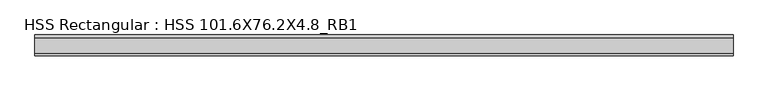
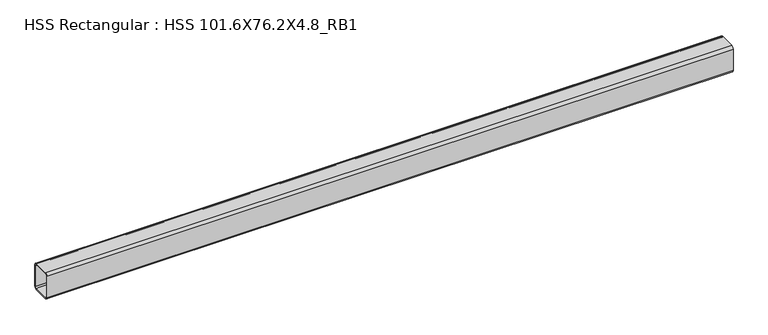
"""IFC4 building model written with IfcOpenShell, lengths in millimetres: beam geometry, HSS Rectangular : HSS 101.6X76.2X4.8_RB1."""

import ifcopenshell
import ifcopenshell.guid

model = None  # the IFC model being written
_history = None  # IfcOwnerHistory: only IFC2X3 demands one
_inside = {}  # id of a spatial element -> (the spatial element, [elements in it])
_under = {}  # id of a project, library or spatial element -> (it, [spatial elements below it])
_declared = {}  # id of a project -> (the project, [libraries it declares])
_typed = {}  # id of a type object -> (the type object, [elements of that type])
_made_of = {}  # id of a material, layer set ... -> (it, [elements and type objects made of it])


def new_model(schema):
    """Start an empty IFC model of exactly this schema.

    Asked for "IFC4X3", IfcOpenShell would pick the latest addendum, in which some entities
    have other attributes; the version numbers below select the first issue.
    IFC2X3 requires an IfcOwnerHistory on every rooted entity: one is made here for all.
    """
    global model, _history
    if schema == "IFC4X3":
        model = ifcopenshell.file(schema_version=(4, 3, 0, 0))
    else:
        model = ifcopenshell.file(schema=schema)
    _inside.clear()
    _under.clear()
    _declared.clear()
    _typed.clear()
    _made_of.clear()
    _history = None
    if model.schema == "IFC2X3":
        org = make("IfcOrganization", Name="unknown")
        user = make(
            "IfcPersonAndOrganization",
            ThePerson=make("IfcPerson", FamilyName="unknown"),
            TheOrganization=org,
        )
        app = make(
            "IfcApplication",
            ApplicationDeveloper=org,
            Version="unknown",
            ApplicationFullName="unknown",
            ApplicationIdentifier="unknown",
        )
        _history = make(
            "IfcOwnerHistory",
            OwningUser=user,
            OwningApplication=app,
            ChangeAction="ADDED",
            CreationDate=0,
        )
    return model


def make(cls, **values):
    """One entity of the class cls with the attributes given. An attribute that is None is left unset."""
    return model.create_entity(
        cls, **{name: value for name, value in values.items() if value is not None}
    )


def rooted(cls, **values):
    """An entity with a GlobalId (a new one), such as an element, a storey or a relation."""
    return make(cls, GlobalId=ifcopenshell.guid.new(), OwnerHistory=_history, **values)


def si_unit(unit_type, name, prefix=None):
    """IfcSIUnit, for example si_unit("LENGTHUNIT", "METRE", prefix="MILLI")."""
    return make("IfcSIUnit", UnitType=unit_type, Prefix=prefix, Name=name)


def assignment(units):
    """IfcUnitAssignment: the units of a project."""
    return None if units is None else make("IfcUnitAssignment", Units=units)


def point(xyz):
    """IfcCartesianPoint."""
    return None if xyz is None else make("IfcCartesianPoint", Coordinates=xyz)


def direction(xyz):
    """IfcDirection."""
    return None if xyz is None else make("IfcDirection", DirectionRatios=xyz)


def frame(location, z_axis=None, x_axis=None):
    """IfcAxis2Placement3D, a coordinate frame: its origin and axes. An axis left out is left unset."""
    return make(
        "IfcAxis2Placement3D",
        Location=point(location),
        Axis=direction(z_axis),
        RefDirection=direction(x_axis),
    )


def frame_2d(location, x_axis=None):
    """IfcAxis2Placement2D, a coordinate frame in the plane: its origin and x axis."""
    return make(
        "IfcAxis2Placement2D", Location=point(location), RefDirection=direction(x_axis)
    )


def origin():
    """The frame at (0, 0, 0) with its axes left unset."""
    return frame((0.0, 0.0, 0.0))


def place(relative_to, where):
    """IfcLocalPlacement: puts the frame where relative to a parent placement (None: the world)."""
    return make(
        "IfcLocalPlacement", PlacementRelTo=relative_to, RelativePlacement=where
    )


def context(
    kind, dimensions, precision=None, world=None, true_north=None, identifier=None
):
    """IfcGeometricRepresentationContext, for example the 3D "Model" context."""
    return make(
        "IfcGeometricRepresentationContext",
        ContextIdentifier=identifier,
        ContextType=kind,
        CoordinateSpaceDimension=dimensions,
        Precision=precision,
        WorldCoordinateSystem=world,
        TrueNorth=true_north,
    )


def project(units=None, contexts=None):
    """IfcProject with its units and contexts."""
    return rooted(
        "IfcProject",
        Name="project",
        RepresentationContexts=contexts,
        UnitsInContext=assignment(units),
    )


def spatial(cls, under=None, at=None, **own):
    """A site, building, storey or space (cls), placed at a placement, below another one or the project."""
    s = rooted(cls, ObjectPlacement=at, **own)
    if under is not None:
        _under.setdefault(under.id(), (under, []))[1].append(s)
    return s


def polyline(points):
    """IfcPolyline through the points."""
    return make("IfcPolyline", Points=[point(p) for p in points])


def circle_curve(where, radius):
    """IfcCircle in the frame where."""
    return make("IfcCircle", Position=where, Radius=radius)


def trimmed(basis, trim1, trim2, sense, master):
    """IfcTrimmedCurve: the piece of a basis curve between two trims."""
    return make(
        "IfcTrimmedCurve",
        BasisCurve=basis,
        Trim1=trim1,
        Trim2=trim2,
        SenseAgreement=sense,
        MasterRepresentation=master,
    )


def segment(curve, same_sense, transition):
    """IfcCompositeCurveSegment."""
    return make(
        "IfcCompositeCurveSegment",
        Transition=transition,
        SameSense=same_sense,
        ParentCurve=curve,
    )


def composite_curve(segments, self_intersect=None):
    """IfcCompositeCurve: segments joined end to end."""
    return make("IfcCompositeCurve", Segments=segments, SelfIntersect=self_intersect)


def outline(outer, holes=None, kind="AREA"):
    """IfcArbitraryClosedProfileDef: a profile drawn as a closed curve; with holes, ...WithVoids."""
    if holes is None:
        return make("IfcArbitraryClosedProfileDef", ProfileType=kind, OuterCurve=outer)
    return make(
        "IfcArbitraryProfileDefWithVoids",
        ProfileType=kind,
        OuterCurve=outer,
        InnerCurves=holes,
    )


def extrude(swept, where, along, depth):
    """IfcExtrudedAreaSolid: the profile swept, set in the frame where, extruded along a direction by depth."""
    return make(
        "IfcExtrudedAreaSolid",
        SweptArea=swept,
        Position=where,
        ExtrudedDirection=direction(along),
        Depth=depth,
    )


def shape(context_of_items, identifier, shape_type, items):
    """IfcShapeRepresentation: the items that make up one representation, for example the "Body"."""
    return make(
        "IfcShapeRepresentation",
        ContextOfItems=context_of_items,
        RepresentationIdentifier=identifier,
        RepresentationType=shape_type,
        Items=items,
    )


def source(mapping_origin, context_of_items, identifier, shape_type, items):
    """IfcRepresentationMap: a shape defined once, which mapped items show again and again."""
    return make(
        "IfcRepresentationMap",
        MappingOrigin=mapping_origin,
        MappedRepresentation=shape(context_of_items, identifier, shape_type, items),
    )


def transform(
    local_origin,
    x_axis=None,
    y_axis=None,
    z_axis=None,
    scale=None,
    scale2=None,
    scale3=None,
    uniform=True,
):
    """IfcCartesianTransformationOperator3D, or its non-uniform kind. x_axis, y_axis, z_axis: its Axis1, 2, 3."""
    if uniform:
        return make(
            "IfcCartesianTransformationOperator3D",
            Axis1=direction(x_axis),
            Axis2=direction(y_axis),
            LocalOrigin=point(local_origin),
            Scale=scale,
            Axis3=direction(z_axis),
        )
    return make(
        "IfcCartesianTransformationOperator3DnonUniform",
        Axis1=direction(x_axis),
        Axis2=direction(y_axis),
        LocalOrigin=point(local_origin),
        Scale=scale,
        Axis3=direction(z_axis),
        Scale2=scale2,
        Scale3=scale3,
    )


def mapped(mapping_source, mapping_target):
    """IfcMappedItem: shows the shape of a source again, moved by a transform."""
    return make(
        "IfcMappedItem", MappingSource=mapping_source, MappingTarget=mapping_target
    )


def made_of(thing, what):
    """Note that an element or type object is made of a material, layer set ...; save() writes the relation."""
    if what is not None:
        _made_of.setdefault(what.id(), (what, []))[1].append(thing)
    return thing


def element(
    cls,
    number,
    at=None,
    inside=None,
    cuts=None,
    type_object=None,
    material=None,
    context=None,
    identifier="Body",
    shape_type=None,
    held_by="IfcProductDefinitionShape",
    body=None,
    shapes=None,
    **own,
):
    """One element of the class cls, such as IfcWall. Its Tag is "e" and its number.

    at: its placement. inside: the storey or other place that contains it. cuts: it is an
    opening in that element (IfcRelVoidsElement). A single representation is given by context,
    identifier, shape_type and body (its items); several are given by shapes. held_by: the class
    of the entity that holds the representations. save() writes the other relations.
    """
    e = rooted(cls, Tag="e%d" % number, ObjectPlacement=at, **own)
    if body is not None:
        shapes = [shape(context, identifier, shape_type, body)]
    if shapes is not None:
        e.Representation = make(held_by, Representations=shapes)
    if inside is not None:
        _inside.setdefault(inside.id(), (inside, []))[1].append(e)
    if cuts is not None:
        rooted(
            "IfcRelVoidsElement", RelatingBuildingElement=cuts, RelatedOpeningElement=e
        )
    if type_object is not None:
        _typed.setdefault(type_object.id(), (type_object, []))[1].append(e)
    return made_of(e, material)


def aggregate(whole, parts):
    """IfcRelAggregates: a whole, such as a stair, and the parts it consists of."""
    return rooted("IfcRelAggregates", RelatingObject=whole, RelatedObjects=parts)


def save(model, path):
    """Write the relations noted so far, then the file.

    IfcRelAggregates (storeys below a building ...), IfcRelContainedInSpatialStructure (elements
    in a storey), IfcRelDefinesByType, IfcRelAssociatesMaterial and IfcRelDeclares: one each for
    every whole, place, type object, material and project.
    """
    for whole, parts in _under.values():
        aggregate(whole, parts)
    for where, things in _inside.values():
        rooted(
            "IfcRelContainedInSpatialStructure",
            RelatedElements=things,
            RelatingStructure=where,
        )
    for kind, things in _typed.values():
        rooted("IfcRelDefinesByType", RelatedObjects=things, RelatingType=kind)
    for what, things in _made_of.values():
        rooted("IfcRelAssociatesMaterial", RelatedObjects=things, RelatingMaterial=what)
    for by, libraries in _declared.values():
        rooted("IfcRelDeclares", RelatingContext=by, RelatedDefinitions=libraries)
    model.write(path)


def hss_rectangular_hss_101_6x76_2x4_8_rb1_f5ecbbfe(model_context):
    return source(origin(), model_context, "Body", "SweptSolid", [
        extrude(outline(composite_curve([segment(polyline([(38.1, 41.275), (38.1, -41.275)]), True, "CONTINUOUS"), segment(trimmed(circle_curve(frame_2d((28.575, -41.275)), 9.525), [point((38.1, -41.275))], [point((28.575, -50.8))], False, "CARTESIAN"), True, "CONTINUOUS"), segment(polyline([(28.575, -50.8), (-28.575, -50.8)]), True, "CONTINUOUS"), segment(trimmed(circle_curve(frame_2d((-28.575, -41.275)), 9.525), [point((-28.575, -50.8))], [point((-38.1, -41.275))], False, "CARTESIAN"), True, "CONTINUOUS"), segment(polyline([(-38.1, -41.275), (-38.1, 41.275)]), True, "CONTINUOUS"), segment(trimmed(circle_curve(frame_2d((-28.575, 41.275)), 9.525), [point((-38.1, 41.275))], [point((-28.575, 50.8))], False, "CARTESIAN"), True, "CONTINUOUS"), segment(polyline([(-28.575, 50.8), (28.575, 50.8)]), True, "CONTINUOUS"), segment(trimmed(circle_curve(frame_2d((28.575, 41.275)), 9.525), [point((28.575, 50.8))], [point((38.1, 41.275))], False, "CARTESIAN"), True, "CONTINUOUS")], self_intersect=False), holes=[composite_curve([segment(trimmed(circle_curve(frame_2d((-28.575, 41.275)), 4.7625), [point((-28.575, 46.0375))], [point((-33.3375, 41.275))], True, "CARTESIAN"), True, "CONTINUOUS"), segment(polyline([(-33.3375, 41.275), (-33.3375, -41.275)]), True, "CONTINUOUS"), segment(trimmed(circle_curve(frame_2d((-28.575, -41.275)), 4.7625), [point((-33.3375, -41.275))], [point((-28.575, -46.0375))], True, "CARTESIAN"), True, "CONTINUOUS"), segment(polyline([(-28.575, -46.0375), (28.575, -46.0375)]), True, "CONTINUOUS"), segment(trimmed(circle_curve(frame_2d((28.575, -41.275)), 4.7625), [point((28.575, -46.0375))], [point((33.3375, -41.275))], True, "CARTESIAN"), True, "CONTINUOUS"), segment(polyline([(33.3375, -41.275), (33.3375, 41.275)]), True, "CONTINUOUS"), segment(trimmed(circle_curve(frame_2d((28.575, 41.275)), 4.7625), [point((33.3375, 41.275))], [point((28.575, 46.0375))], True, "CARTESIAN"), True, "CONTINUOUS"), segment(polyline([(28.575, 46.0375), (-28.575, 46.0375)]), True, "CONTINUOUS")], self_intersect=False)]), frame((-1267.75, 0.0, 0.0), z_axis=(1.0, 0.0, 0.0), x_axis=(0.0, 1.0, 0.0)), (0.0, 0.0, 1.0), 2535.5),
    ])


if __name__ == "__main__":
    model = new_model("IFC4")
    model_context = context("Model", 3, world=origin())
    ifc_project = project(units=[si_unit("LENGTHUNIT", "METRE", prefix="MILLI")], contexts=[model_context])
    site = spatial("IfcSite", under=ifc_project)
    building = spatial("IfcBuilding", under=site)
    placement = place(None, origin())
    hss_rectangular_hss_101_6x76_2x4_8_rb1_shape = hss_rectangular_hss_101_6x76_2x4_8_rb1_f5ecbbfe(model_context)
    element("IfcBeam", 1, ObjectType="HSS Rectangular : HSS 101.6X76.2X4.8_RB1", at=placement, inside=building, context=model_context, shape_type="MappedRepresentation", body=[
        mapped(hss_rectangular_hss_101_6x76_2x4_8_rb1_shape, transform((0.0, 0.0, 0.0), x_axis=(1.0, 0.0, 0.0), y_axis=(0.0, 1.0, 0.0), z_axis=(0.0, 0.0, 1.0))),
    ])
    save(model, "model.ifc")

# Revit data of these elements
# Type "HSS Rectangular : HSS 101.6X76.2X4.8_RB1"
#   Section Name Key = "HSS 4X3X3/16"
#   Assembly Code = "B10"
#   Width = 7.62 cm
#   Wall Nominal Thickness = 0.4763 cm
#   Wall Design Thickness = 0.442 cm
#   Torsional Moment of Inertia = 260.561 cm⁴
#   Torsional Modulus = 61.2876 cm³
#   Section Area = 14.4516 cm²
#   Plastic Modulus weak axis = 40.3122 cm³
#   Plastic Modulus strong axis = 49.1612 cm³
#   Perimeter = 0.881482 m²/m
#   Outer Fillet = 0.9525 cm
#   Nominal Weight = 12.1285 kgf/m
#   Moment of Inertia weak axis = 131.529 cm⁴
#   Moment of Inertia strong axis = 205.202 cm⁴
#   Inner Fillet = 0.4763 cm
#   Height = 10.16 cm
#   Elastic Modulus weak axis = 34.4128 cm³
#   Elastic Modulus strong axis = 40.476 cm³
#   Centroid Vertical = 5.08 cm
#   Centroid Horizontal = 3.81 cm
#   Length [instance default] = 1524 mm
#   Structural Material [instance default] = Steel ASTM A500, Grade B, Rectangular and Square
#   Principal Axes Angle = 0
# Element 1 (IfcBeam, "HSS Rectangular : HSS 101.6X76.2X4.8_RB1")
#   Structural Material = Steel ASTM A992
#   Materials on its faces: "Steel ASTM A992"
# Materials
#   "Steel ASTM A500, Grade B, Rectangular and Square": class "Metal", colour RGB 199 199 199, transparency 0, Description = "Carbon steel", Cost = 0
#   "Steel ASTM A992": class "Metal", colour RGB 199 199 199, transparency 0, Description = "Structural steel 50ksi", Cost = 0
